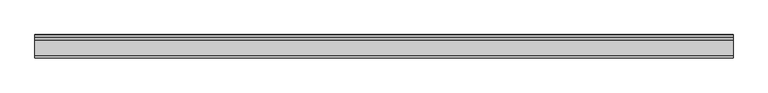
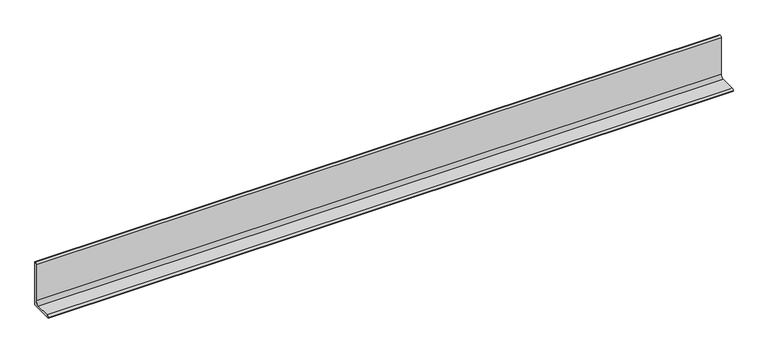
"""IFC4 building model written with IfcOpenShell, lengths in millimetres: beam geometry, NLRS_28_SF_LIB_stalen ligger hoekprofiel ongelijkzijdig-AV-MMBS-SRP_gen_rsf : stalen ligger ongelijzijdig hoekprofiel LUEQ_gen__200x100x10."""

from ifc_helpers import new_model, si_unit, point, frame, frame_2d, origin, place, context, project, spatial, polyline, circle_curve, trimmed, segment, composite_curve, outline, extrude, source, transform, mapped, element, save


def beam_42ca15b0(model_context):
    return source(origin(), model_context, "Body", "SweptSolid", [
        extrude(outline(composite_curve([segment(polyline([(20.13, -69.3), (-79.87, -69.3), (-79.87, -66.8)]), True, "CONTINUOUS"), segment(trimmed(circle_curve(frame_2d((-72.37, -66.8)), 7.5), [point((-79.87, -66.8))], [point((-72.37, -59.3))], False, "CARTESIAN"), True, "CONTINUOUS"), segment(polyline([(-72.37, -59.3), (-4.87, -59.3)]), True, "CONTINUOUS"), segment(trimmed(circle_curve(frame_2d((-4.87, -44.3)), 15.0), [point((-4.87, -59.3))], [point((10.13, -44.3))], True, "CARTESIAN"), True, "CONTINUOUS"), segment(polyline([(10.13, -44.3), (10.13, 123.2)]), True, "CONTINUOUS"), segment(trimmed(circle_curve(frame_2d((17.63, 123.2)), 7.5), [point((10.13, 123.2))], [point((17.63, 130.7))], False, "CARTESIAN"), True, "CONTINUOUS"), segment(polyline([(17.63, 130.7), (20.13, 130.7), (20.13, -69.3)]), True, "CONTINUOUS")], self_intersect=False)), frame((-1500.0, 0.0, 0.0), z_axis=(1.0, 0.0, 0.0), x_axis=(0.0, 1.0, 0.0)), (0.0, 0.0, 1.0), 3000.0),
    ])


if __name__ == "__main__":
    model = new_model("IFC4")
    model_context = context("Model", 3, world=origin())
    ifc_project = project(units=[si_unit("LENGTHUNIT", "METRE", prefix="MILLI")], contexts=[model_context])
    site = spatial("IfcSite", under=ifc_project)
    building = spatial("IfcBuilding", under=site)
    placement = place(None, origin())
    beam_shape = beam_42ca15b0(model_context)
    element("IfcBeam", 1, ObjectType="NLRS_28_SF_LIB_stalen ligger hoekprofiel ongelijkzijdig-AV-MMBS-SRP_gen_rsf : stalen ligger ongelijzijdig hoekprofiel LUEQ_gen__200x100x10", at=placement, inside=building, context=model_context, shape_type="MappedRepresentation", body=[
        mapped(beam_shape, transform((0.0, 0.0, 0.0), x_axis=(1.0, 0.0, 0.0), y_axis=(0.0, 1.0, 0.0), z_axis=(0.0, 0.0, 1.0))),
    ])
    save(model, "model.ifc")

# Revit data of these elements
# Type "NLRS_28_SF_LIB_stalen ligger hoekprofiel ongelijkzijdig-AV-MMBS-SRP_gen_rsf : stalen ligger ongelijzijdig hoekprofiel LUEQ_gen__200x100x10"
#   Type IfcGUID = "0dxhH9VHH5jh7XQ0uLfXuR"
#   IfcExportAs = "IfcBeamType"
#   Type Comments = "L200x100x10"
#   Model = " "
#   Manufacturer = " "
#   Fire Rating = " "
#   Description = "stalen ligger L200x100x10"
#   Assembly Code = "28.11"
#   vz = 130.7 mm
#   vy = 79.87 mm
#   tw = 10 mm
#   tf = 10 mm
#   ri = 7.5 mm
#   ra = 15 mm
#   d = 200 mm
#   bf = 100 mm
#   NLRS_C_lengte [instance default] = 1524 mm
#   Length [instance default] = 1524 mm
#   Structural Material = NLRS_h2_staal_gen_rsf
#   Keynote = ""
# Element 1 (IfcBeam, "NLRS_28_SF_LIB_stalen ligger hoekprofiel ongelijkzijdig-AV-MMBS-SRP_gen_rsf : stalen ligger ongelijzijdig hoekprofiel LUEQ_gen__200x100x10")
#   NLRS_C_lengte = 3000 mm
#   Materials on its faces: "NLRS_h2_staal_gen_rsf"
# Materials
#   "NLRS_h2_staal_gen_rsf": class "H - Metaal", colour RGB 189 187 185, transparency 0, Keynote = "h2", Manufacturer = "Revit Standards Foundation", URL = "www.revitstandards.org", Description = "staal", Cost = 0
